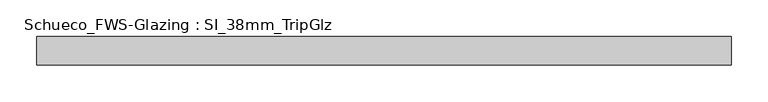
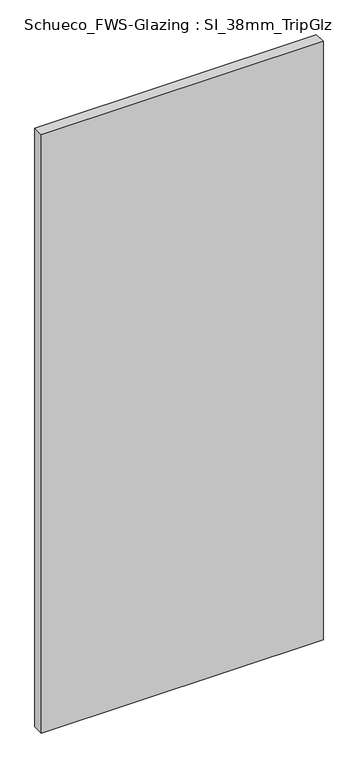
"""IFC4 building model written with IfcOpenShell, lengths in millimetres: plate geometry, Schueco_FWS-Glazing : SI_38mm_TripGlz."""

from ifc_helpers import new_model, si_unit, origin, origin_with_axes, place, context, project, spatial, polyline, outline, extrude, source, transform, mapped, element, save


def schueco_fws_glazing_si_38mm_tripglz_9e1f98aa(model_context):
    return source(origin(), model_context, "Body", "SweptSolid", [
        extrude(outline(polyline([(469.0, -38.0), (-469.0, -38.0), (-469.0, 0.0), (469.0, 0.0), (469.0, -38.0)])), origin_with_axes(), (0.0, 0.0, 1.0), 2108.0),
    ])


if __name__ == "__main__":
    model = new_model("IFC4")
    model_context = context("Model", 3, world=origin())
    ifc_project = project(units=[si_unit("LENGTHUNIT", "METRE", prefix="MILLI")], contexts=[model_context])
    site = spatial("IfcSite", under=ifc_project)
    building = spatial("IfcBuilding", under=site)
    placement = place(None, origin())
    schueco_fws_glazing_si_38mm_tripglz_shape = schueco_fws_glazing_si_38mm_tripglz_9e1f98aa(model_context)
    element("IfcPlate", 1, ObjectType="Schueco_FWS-Glazing : SI_38mm_TripGlz", at=placement, inside=building, context=model_context, shape_type="MappedRepresentation", body=[
        mapped(schueco_fws_glazing_si_38mm_tripglz_shape, transform((0.0, 0.0, 0.0), x_axis=(1.0, 0.0, 0.0), y_axis=(0.0, 1.0, 0.0), z_axis=(0.0, 0.0, 1.0))),
    ])
    save(model, "model.ifc")

# Revit data of these elements
# Type "Schueco_FWS-Glazing : SI_38mm_TripGlz"
#   Model = "Triple glazing 38mm"
#   Manufacturer = "Schueco International KG"
#   Analytic Construction = "<Keine Auswahl>"
#   Glazing thickness = 38 mm
#   FWS SI insert unit = yes
#   FWS HI insert unit = no
#   Glass = Glass
# Element 1 (IfcPlate, "Schueco_FWS-Glazing : SI_38mm_TripGlz")
#   Materials on its faces: "Glass"
# Materials
#   "Glass": class "Glass", colour RGB 128 128 255, transparency 0.75, Description = "Soda Lime Glass", Cost = 0
